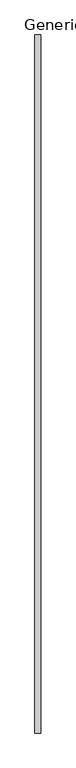
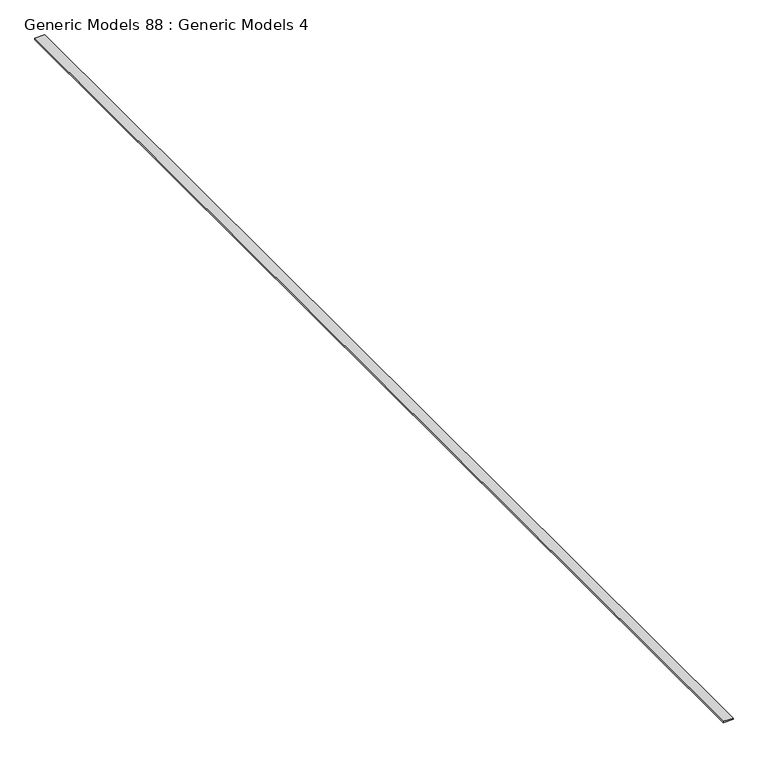
"""IFC4 building model written with IfcOpenShell, lengths in millimetres: proxy geometry, Generic Models 88 : Generic Models 4."""

from ifc_helpers import new_model, si_unit, frame, origin, place, context, project, spatial, polyline, outline, extrude, source, transform, mapped, element, save


def generic_models_88_generic_models_4_f8f801a1(model_context):
    return source(origin(), model_context, "Body", "SweptSolid", [
        extrude(outline(polyline([(7243.9063704, -6864.9230338), (7087.6963704, -6864.9230338), (7087.6963704, 11778.6769662), (7243.9063704, 11778.6769662), (7243.9063704, -6864.9230338)])), frame((0.0, 0.0, 126304.421), z_axis=(0.0, 0.0, 1.0), x_axis=(1.0, 0.0, 0.0)), (0.0, 0.0, 1.0), 22.225),
    ])


if __name__ == "__main__":
    model = new_model("IFC4")
    model_context = context("Model", 3, world=origin())
    ifc_project = project(units=[si_unit("LENGTHUNIT", "METRE", prefix="MILLI")], contexts=[model_context])
    site = spatial("IfcSite", under=ifc_project)
    building = spatial("IfcBuilding", under=site)
    placement = place(None, origin())
    generic_models_88_generic_models_4_shape = generic_models_88_generic_models_4_f8f801a1(model_context)
    element("IfcBuildingElementProxy", 1, Name="Generic Models 88 : Generic Models 4", ObjectType="Generic Models 88 : Generic Models 4", at=placement, inside=building, context=model_context, shape_type="MappedRepresentation", body=[
        mapped(generic_models_88_generic_models_4_shape, transform((0.0, 0.0, 0.0), x_axis=(1.0, 0.0, 0.0), y_axis=(0.0, 1.0, 0.0), z_axis=(0.0, 0.0, 1.0))),
    ])
    save(model, "model.ifc")

# Revit data of these elements
# Element 1 (IfcBuildingElementProxy, "Generic Models 88 : Generic Models 4")
#   Materials on its faces: "_7/8\" SMOOTH TROWEL EXTERIOR STUCCO (COLOR PER OWNER)"
# Materials
#   "_7/8\" SMOOTH TROWEL EXTERIOR STUCCO (COLOR PER OWNER)": class "Generic", colour RGB 233 233 233, transparency 0, Cost = 0
